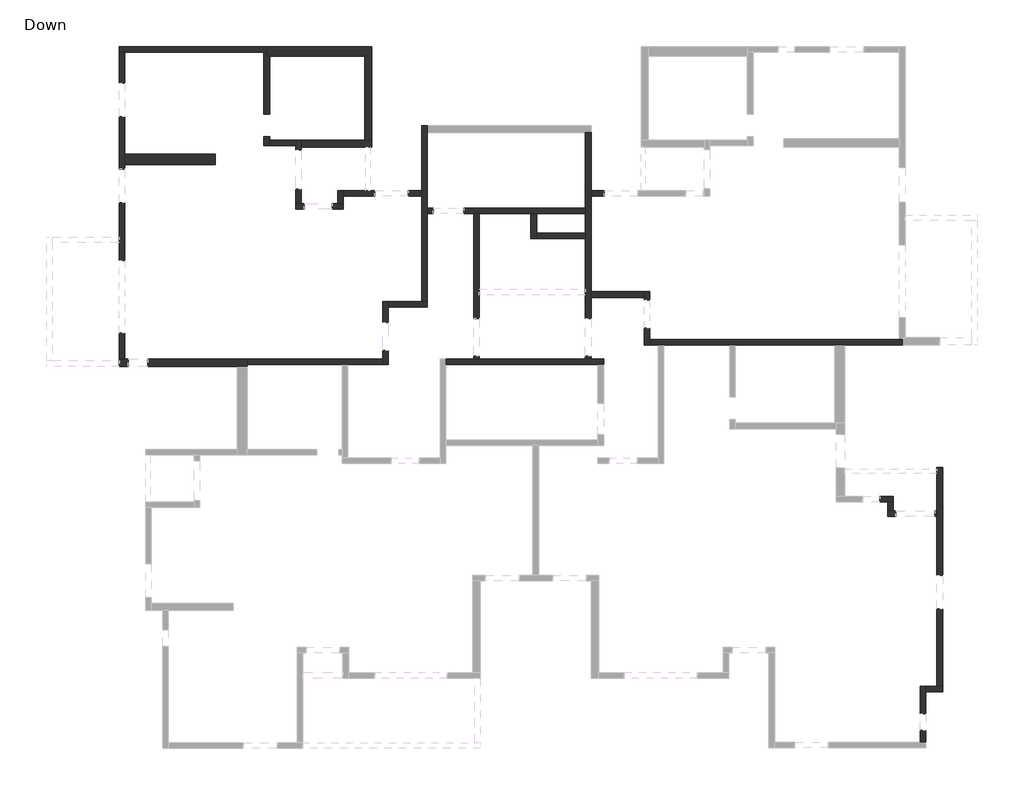
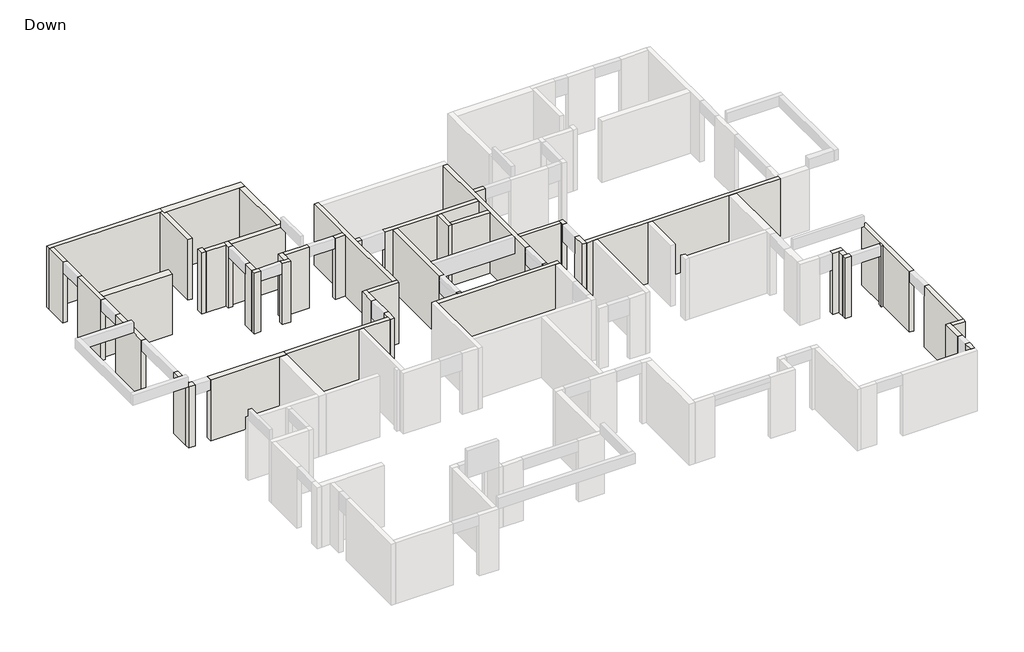
# One storey, part 2 of 3: 49 walls.
# Revit data of these elements (continued)
# Element 30 (IfcWall, "20")
#   Comments = ""
#   Mark = "W72"
#   SOFiSTiK_EdgeZones = "W72"
#   SOFiSTiK_AMG_Comments = ""
#   Top Offset = 0 cm
#   Base Offset = 0 cm
#   wall height = 300 cm
#   SOFiSTiK_AMG_Scheduled = yes
#   SOFiSTiK_AMG_Adjusted = yes
#   Phase Created = New Construction
#   Base Constraint = Down
#   Top Constraint = Typical Floor
#   Materials on its faces: "Concrete"
# Element 31 (IfcWall, "20")
#   Comments = ""
#   Mark = "W73"
#   SOFiSTiK_EdgeZones = "W73"
#   SOFiSTiK_AMG_Comments = ""
#   Top Offset = 0 cm
#   Base Offset = 0 cm
#   wall height = 300 cm
#   SOFiSTiK_AMG_Scheduled = yes
#   SOFiSTiK_AMG_Adjusted = yes
#   Phase Created = New Construction
#   Base Constraint = Down
#   Top Constraint = Typical Floor
#   Materials on its faces: "Concrete"
# Element 32 (IfcWall, "20")
#   Comments = ""
#   Mark = "W74"
#   SOFiSTiK_EdgeZones = "W74"
#   SOFiSTiK_AMG_Comments = ""
#   Top Offset = 0 cm
#   Base Offset = 0 cm
#   wall height = 300 cm
#   SOFiSTiK_AMG_Scheduled = yes
#   SOFiSTiK_AMG_Adjusted = yes
#   Phase Created = New Construction
#   Base Constraint = Down
#   Top Constraint = Typical Floor
#   Materials on its faces: "Concrete"
# Element 33 (IfcWall, "20")
#   Comments = ""
#   Mark = "W75"
#   SOFiSTiK_EdgeZones = "W75"
#   SOFiSTiK_AMG_Comments = ""
#   Top Offset = 0 cm
#   Base Offset = 0 cm
#   wall height = 300 cm
#   SOFiSTiK_AMG_Scheduled = yes
#   SOFiSTiK_AMG_Adjusted = yes
#   Phase Created = New Construction
#   Base Constraint = Down
#   Top Constraint = Typical Floor
#   Materials on its faces: "Concrete"
# Element 34 (IfcWall, "20")
#   Comments = ""
#   Mark = "W76"
#   SOFiSTiK_EdgeZones = "W76"
#   SOFiSTiK_AMG_Comments = "Too Short /"
#   Top Offset = 0 cm
#   Base Offset = 0 cm
#   wall height = 300 cm
#   SOFiSTiK_AMG_Scheduled = yes
#   SOFiSTiK_AMG_Adjusted = yes
#   Phase Created = New Construction
#   Base Constraint = Down
#   Top Constraint = Typical Floor
#   Materials on its faces: "Concrete"
# Element 35 (IfcWall, "20")
#   Comments = ""
#   Mark = "W77"
#   SOFiSTiK_EdgeZones = "W77"
#   SOFiSTiK_AMG_Comments = ""
#   Top Offset = 0 cm
#   Base Offset = 0 cm
#   wall height = 300 cm
#   SOFiSTiK_AMG_Scheduled = yes
#   SOFiSTiK_AMG_Adjusted = yes
#   Phase Created = New Construction
#   Base Constraint = Down
#   Top Constraint = Typical Floor
#   Materials on its faces: "Concrete"
# Element 36 (IfcWall, "20")
#   Comments = ""
#   Mark = "W78"
#   SOFiSTiK_EdgeZones = "W78"
#   SOFiSTiK_AMG_Comments = ""
#   Top Offset = 0 cm
#   Base Offset = 0 cm
#   wall height = 300 cm
#   SOFiSTiK_AMG_Scheduled = yes
#   SOFiSTiK_AMG_Adjusted = yes
#   Phase Created = New Construction
#   Base Constraint = Down
#   Top Constraint = Typical Floor
#   Materials on its faces: "Concrete"
# Element 37 (IfcWall, "20")
#   Comments = ""
#   Mark = "W79"
#   SOFiSTiK_EdgeZones = "W79"
#   SOFiSTiK_AMG_Comments = ""
#   Top Offset = 0 cm
#   Base Offset = 0 cm
#   wall height = 300 cm
#   SOFiSTiK_AMG_Scheduled = yes
#   SOFiSTiK_AMG_Adjusted = yes
#   Phase Created = New Construction
#   Base Constraint = Down
#   Top Constraint = Typical Floor
#   Materials on its faces: "Concrete"
# Element 38 (IfcWall, "20")
#   Comments = ""
#   Mark = "W85"
#   SOFiSTiK_EdgeZones = "W85"
#   SOFiSTiK_AMG_Comments = ""
#   Top Offset = 0 cm
#   Base Offset = 0 cm
#   wall height = 300 cm
#   SOFiSTiK_AMG_Scheduled = yes
#   SOFiSTiK_AMG_Adjusted = yes
#   Phase Created = New Construction
#   Base Constraint = Down
#   Top Constraint = Typical Floor
#   Materials on its faces: "Concrete"
# Element 39 (IfcWall, "20")
#   Comments = ""
#   Mark = "W86"
#   SOFiSTiK_EdgeZones = "W86"
#   SOFiSTiK_AMG_Comments = ""
#   Top Offset = 0 cm
#   Base Offset = 0 cm
#   wall height = 300 cm
#   SOFiSTiK_AMG_Scheduled = yes
#   SOFiSTiK_AMG_Adjusted = yes
#   Phase Created = New Construction
#   Base Constraint = Down
#   Top Constraint = Typical Floor
#   Materials on its faces: "Concrete"
# Element 40 (IfcWall, "20")
#   Comments = ""
#   Mark = "W100"
#   SOFiSTiK_EdgeZones = "W100"
#   SOFiSTiK_AMG_Comments = ""
#   Top Offset = 0 cm
#   Base Offset = 0 cm
#   wall height = 300 cm
#   SOFiSTiK_AMG_Scheduled = yes
#   SOFiSTiK_AMG_Adjusted = yes
#   Phase Created = New Construction
#   Base Constraint = Down
#   Top Constraint = Typical Floor
#   Materials on its faces: "Concrete"
# Element 41 (IfcWall, "20")
#   Comments = ""
#   Mark = "W105"
#   SOFiSTiK_EdgeZones = "W105"
#   SOFiSTiK_AMG_Comments = "Too Short /"
#   Top Offset = 0 cm
#   Base Offset = 0 cm
#   wall height = 300 cm
#   SOFiSTiK_AMG_Scheduled = yes
#   SOFiSTiK_AMG_Adjusted = yes
#   Phase Created = New Construction
#   Base Constraint = Down
#   Top Constraint = Typical Floor
#   Materials on its faces: "Concrete"
# Element 42 (IfcWall, "20")
#   Comments = ""
#   Mark = "W106"
#   SOFiSTiK_EdgeZones = "W106"
#   SOFiSTiK_AMG_Comments = ""
#   Top Offset = 0 cm
#   Base Offset = 0 cm
#   wall height = 300 cm
#   SOFiSTiK_AMG_Scheduled = yes
#   SOFiSTiK_AMG_Adjusted = yes
#   Phase Created = New Construction
#   Base Constraint = Down
#   Top Constraint = Typical Floor
#   Materials on its faces: "Concrete"
# Element 43 (IfcWall, "20")
#   Comments = ""
#   Mark = "W107"
#   SOFiSTiK_EdgeZones = "W107"
#   SOFiSTiK_AMG_Comments = ""
#   Top Offset = 0 cm
#   Base Offset = 0 cm
#   wall height = 300 cm
#   SOFiSTiK_AMG_Scheduled = yes
#   SOFiSTiK_AMG_Adjusted = yes
#   Phase Created = New Construction
#   Base Constraint = Down
#   Top Constraint = Typical Floor
#   Materials on its faces: "Concrete"
# Element 44 (IfcWall, "25")
#   Comments = ""
#   Mark = "W113"
#   SOFiSTiK_EdgeZones = "W113"
#   SOFiSTiK_AMG_Comments = ""
#   Top Offset = 0 cm
#   Base Offset = 0 cm
#   wall height = 300 cm
#   SOFiSTiK_AMG_Scheduled = yes
#   SOFiSTiK_AMG_Adjusted = yes
#   Phase Created = New Construction
#   Base Constraint = Down
#   Top Constraint = Typical Floor
#   Materials on its faces: "Concrete"
# Element 45 (IfcWall, "25")
#   Comments = ""
#   Mark = "W114"
#   SOFiSTiK_EdgeZones = "W114"
#   SOFiSTiK_AMG_Comments = ""
#   Top Offset = 0 cm
#   Base Offset = 0 cm
#   wall height = 300 cm
#   SOFiSTiK_AMG_Scheduled = yes
#   SOFiSTiK_AMG_Adjusted = yes
#   Phase Created = New Construction
#   Base Constraint = Down
#   Top Constraint = Typical Floor
#   Materials on its faces: "Concrete"
# Element 46 (IfcWall, "27")
#   Comments = ""
#   Mark = "W108"
#   SOFiSTiK_EdgeZones = "W108"
#   SOFiSTiK_AMG_Comments = ""
#   Top Offset = 0 cm
#   Base Offset = 0 cm
#   wall height = 300 cm
#   SOFiSTiK_AMG_Scheduled = yes
#   SOFiSTiK_AMG_Adjusted = yes
#   Phase Created = New Construction
#   Base Constraint = Down
#   Top Constraint = Typical Floor
#   Materials on its faces: "Concrete"
# Element 47 (IfcWall, "27")
#   Comments = ""
#   Mark = "W109"
#   SOFiSTiK_EdgeZones = "W109"
#   SOFiSTiK_AMG_Comments = ""
#   Top Offset = 0 cm
#   Base Offset = 0 cm
#   wall height = 300 cm
#   SOFiSTiK_AMG_Scheduled = yes
#   SOFiSTiK_AMG_Adjusted = yes
#   Phase Created = New Construction
#   Base Constraint = Down
#   Top Constraint = Typical Floor
#   Materials on its faces: "Concrete"
# Element 48 (IfcWall, "35")
#   Comments = ""
#   Mark = "W1"
#   SOFiSTiK_EdgeZones = "W1"
#   SOFiSTiK_AMG_Comments = ""
#   Top Offset = 0 cm
#   Base Offset = 0 cm
#   wall height = 300 cm
#   SOFiSTiK_AMG_Scheduled = yes
#   SOFiSTiK_AMG_Adjusted = yes
#   Phase Created = New Construction
#   Base Constraint = Down
#   Top Constraint = Typical Floor
#   Materials on its faces: "Concrete"
# Element 49 (IfcWall, "36")
#   Comments = ""
#   Mark = "W119"
#   SOFiSTiK_EdgeZones = "W119"
#   SOFiSTiK_AMG_Comments = ""
#   Top Offset = 0 cm
#   Base Offset = 0 cm
#   wall height = 300 cm
#   SOFiSTiK_AMG_Scheduled = yes
#   SOFiSTiK_AMG_Adjusted = yes
#   Phase Created = New Construction
#   Base Constraint = Down
#   Top Constraint = Typical Floor
#   Materials on its faces: "Concrete"
# Materials
#   "Concrete": class "Concrete", colour RGB 192 192 192, transparency 0, Keynote = "01000", Description = "Cast-in-place concrete", Cost = 0
